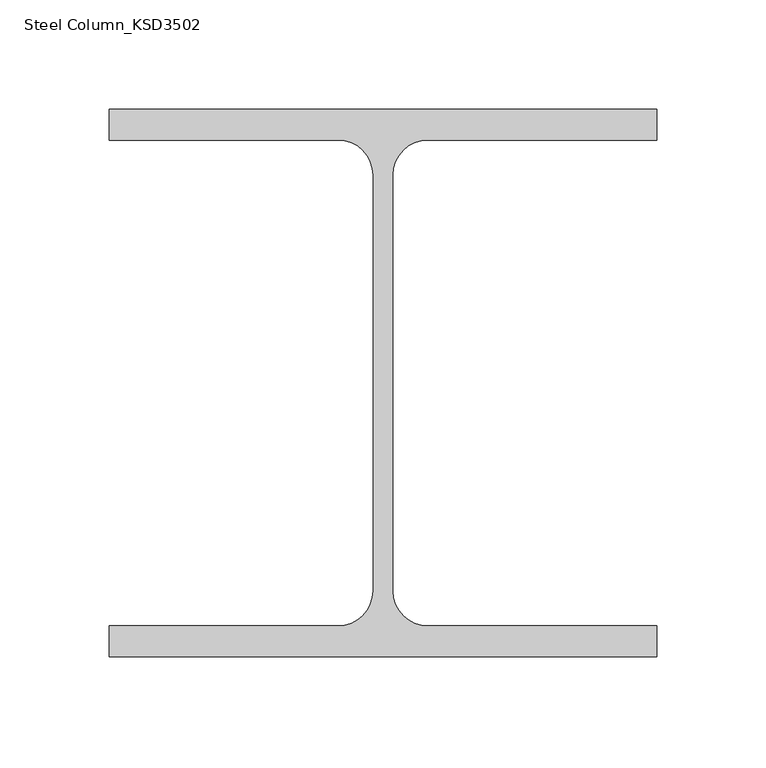
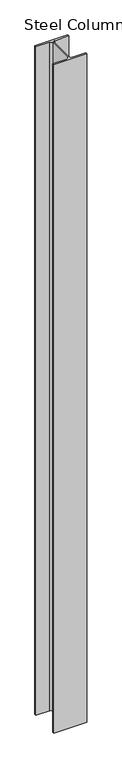
"""IFC4 building model written with IfcOpenShell, lengths in millimetres: column geometry, Steel Column_KSD3502 : H_SC_ASC_H-250×250x9x14."""

from ifc_helpers import new_model, si_unit, point, frame, frame_2d, origin, place, context, project, spatial, polyline, circle_curve, trimmed, segment, composite_curve, outline, extrude, source, transform, mapped, element, save


def steel_column_ksd3502_c81c4db5(model_context):
    return source(origin(), model_context, "Body", "SweptSolid", [
        extrude(outline(composite_curve([segment(polyline([(125.0, 125.0), (125.0, 111.0), (20.5, 111.0)]), True, "CONTINUOUS"), segment(trimmed(circle_curve(frame_2d((20.5, 95.0)), 16.0), [point((20.5, 111.0))], [point((4.5, 95.0))], True, "CARTESIAN"), True, "CONTINUOUS"), segment(polyline([(4.5, 95.0), (4.5, -95.0)]), True, "CONTINUOUS"), segment(trimmed(circle_curve(frame_2d((20.5, -95.0)), 16.0), [point((4.5, -95.0))], [point((20.5, -111.0))], True, "CARTESIAN"), True, "CONTINUOUS"), segment(polyline([(20.5, -111.0), (125.0, -111.0), (125.0, -125.0), (-125.0, -125.0), (-125.0, -111.0), (-20.5, -111.0)]), True, "CONTINUOUS"), segment(trimmed(circle_curve(frame_2d((-20.5, -95.0)), 16.0), [point((-20.5, -111.0))], [point((-4.5, -95.0))], True, "CARTESIAN"), True, "CONTINUOUS"), segment(polyline([(-4.5, -95.0), (-4.5, 95.0)]), True, "CONTINUOUS"), segment(trimmed(circle_curve(frame_2d((-20.5, 95.0)), 16.0), [point((-4.5, 95.0))], [point((-20.5, 111.0))], True, "CARTESIAN"), True, "CONTINUOUS"), segment(polyline([(-20.5, 111.0), (-125.0, 111.0), (-125.0, 125.0), (125.0, 125.0)]), True, "CONTINUOUS")], self_intersect=False)), frame((0.0, 0.0, 599.9720055), z_axis=(0.0, 0.0, 1.0), x_axis=(1.0, 0.0, 0.0)), (0.0, 0.0, 1.0), 5350.0),
    ])


if __name__ == "__main__":
    model = new_model("IFC4")
    model_context = context("Model", 3, world=origin())
    ifc_project = project(units=[si_unit("LENGTHUNIT", "METRE", prefix="MILLI")], contexts=[model_context])
    site = spatial("IfcSite", under=ifc_project)
    building = spatial("IfcBuilding", under=site)
    placement = place(None, origin())
    steel_column_ksd3502_shape = steel_column_ksd3502_c81c4db5(model_context)
    element("IfcColumn", 1, ObjectType="Steel Column_KSD3502 : H_SC_ASC_H-250×250x9x14", at=placement, inside=building, context=model_context, shape_type="MappedRepresentation", body=[
        mapped(steel_column_ksd3502_shape, transform((0.0, 0.0, 0.0), x_axis=(1.0, 0.0, 0.0), y_axis=(0.0, 1.0, 0.0), z_axis=(0.0, 0.0, 1.0))),
    ])
    save(model, "model.ifc")

# Revit data of these elements
# Type "Steel Column_KSD3502 : H_SC_ASC_H-250×250x9x14"
#   Width = 25.0 cm
#   Web Thickness = 0.9 cm
#   Web Fillet = 1.6 cm
#   Warping Constant = 507646.0 cm⁶
#   Torsional Moment of Inertia = 51.4681 cm⁴
#   Section Area = 92.18 cm²
#   Plastic Modulus weak axis = 444.0 cm³
#   Plastic Modulus strong axis = 960.0 cm³
#   Perimeter = 1.27 m²/m
#   Nominal Weight = 72.40 kgf/m
#   Moment of Inertia weak axis = 3650.00 cm⁴
#   Moment of Inertia strong axis = 10800.00 cm⁴
#   Height = 25.0 cm
#   Flange Thickness = 1.4 cm
#   Elastic Modulus weak axis = 292.0 cm³
#   Elastic Modulus strong axis = 867.0 cm³
#   Centroid Vertical = 12.5 cm
#   Centroid Horizontal = 12.5 cm
#   Bolt Spacing = 13.97 cm
#   Structural Material [instance default] = Steel, 45-345
#   Section Name Key = ""
#   Assembly Code = ""
# Element 1 (IfcColumn, "Steel Column_KSD3502 : H_SC_ASC_H-250×250x9x14")
#   Structural Material = A03AD029-00005_Anchor Bolt (Installation only)_M24
#   Materials on its faces: "A03AD029-00005_Anchor Bolt (Installation only)_M24"
# Materials
#   "Steel, 45-345": class "Metal", colour RGB 189 187 185, transparency 0, Description = "Steel 345 MPa", Cost = 0
#   "A03AD029-00005_Anchor Bolt (Installation only)_M24": class "Unassigned", colour RGB 84 83 81, transparency 0, Cost = 0
